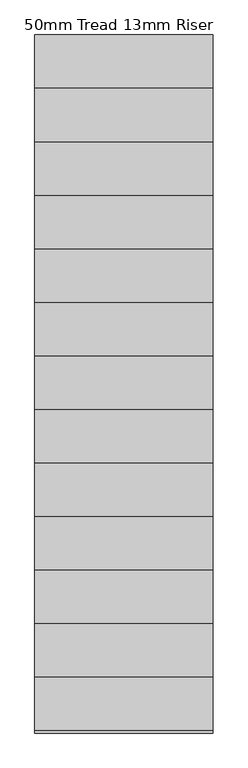
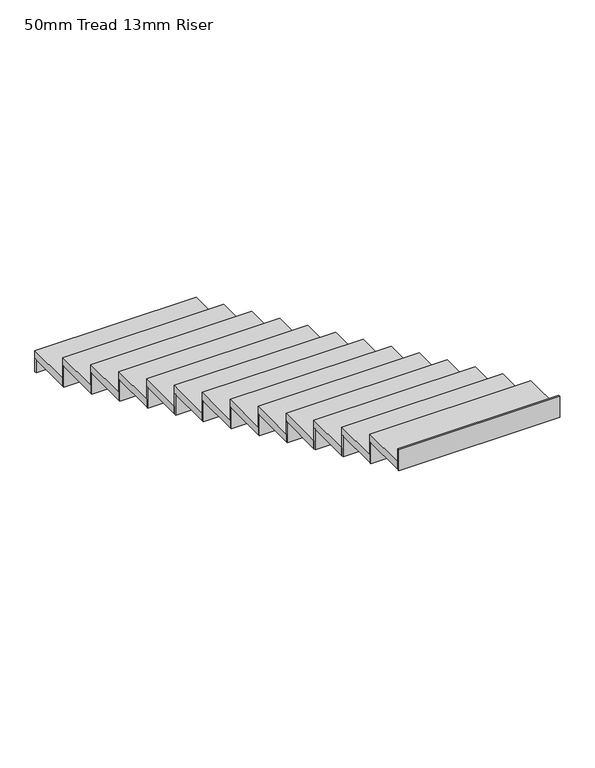
"""IFC4 building model written with IfcOpenShell, lengths in millimetres: stair flight geometry, 50mm Tread 13mm Riser."""

from ifc_helpers import new_model, si_unit, frame, origin, origin_with_axes, place, context, project, spatial, polyline, outline, extrude, source, transform, mapped, element, save


def stair_flight_50mm_tread_13mm_riser_fee8950f(model_context):
    return source(origin(), model_context, "Body", "SweptSolid", [
        extrude(outline(polyline([(-14281.6736899, 1715.8603727), (-14281.6736899, 1728.3603727), (-13281.6736899, 1728.3603727), (-13281.6736899, 1715.8603727), (-14281.6736899, 1715.8603727)])), origin_with_axes(), (0.0, 0.0, 1.0), 86.3636364),
        extrude(outline(polyline([(-13281.6736899, 1428.3603727), (-14281.6736899, 1428.3603727), (-14281.6736899, 1728.3603727), (-13281.6736899, 1728.3603727), (-13281.6736899, 1428.3603727)])), frame((0.0, 0.0, 86.3636364), z_axis=(0.0, 0.0, 1.0), x_axis=(1.0, 0.0, 0.0)), (0.0, 0.0, 1.0), 50.0),
        extrude(outline(polyline([(-14281.6736899, 1415.8603727), (-14281.6736899, 1428.3603727), (-13281.6736899, 1428.3603727), (-13281.6736899, 1415.8603727), (-14281.6736899, 1415.8603727)])), frame((0.0, 0.0, 86.3636364), z_axis=(0.0, 0.0, 1.0), x_axis=(1.0, 0.0, 0.0)), (0.0, 0.0, 1.0), 136.3636364),
        extrude(outline(polyline([(-13281.6736899, 1128.3603727), (-14281.6736899, 1128.3603727), (-14281.6736899, 1428.3603727), (-13281.6736899, 1428.3603727), (-13281.6736899, 1128.3603727)])), frame((0.0, 0.0, 222.7272727), z_axis=(0.0, 0.0, 1.0), x_axis=(1.0, 0.0, 0.0)), (0.0, 0.0, 1.0), 50.0),
        extrude(outline(polyline([(-14281.6736899, 1115.8603727), (-14281.6736899, 1128.3603727), (-13281.6736899, 1128.3603727), (-13281.6736899, 1115.8603727), (-14281.6736899, 1115.8603727)])), frame((0.0, 0.0, 222.7272727), z_axis=(0.0, 0.0, 1.0), x_axis=(1.0, 0.0, 0.0)), (0.0, 0.0, 1.0), 136.3636364),
        extrude(outline(polyline([(-13281.6736899, 828.3603727), (-14281.6736899, 828.3603727), (-14281.6736899, 1128.3603727), (-13281.6736899, 1128.3603727), (-13281.6736899, 828.3603727)])), frame((0.0, 0.0, 359.0909091), z_axis=(0.0, 0.0, 1.0), x_axis=(1.0, 0.0, 0.0)), (0.0, 0.0, 1.0), 50.0),
        extrude(outline(polyline([(-14281.6736899, 815.8603727), (-14281.6736899, 828.3603727), (-13281.6736899, 828.3603727), (-13281.6736899, 815.8603727), (-14281.6736899, 815.8603727)])), frame((0.0, 0.0, 359.0909091), z_axis=(0.0, 0.0, 1.0), x_axis=(1.0, 0.0, 0.0)), (0.0, 0.0, 1.0), 136.3636364),
        extrude(outline(polyline([(-13281.6736899, 528.3603727), (-14281.6736899, 528.3603727), (-14281.6736899, 828.3603727), (-13281.6736899, 828.3603727), (-13281.6736899, 528.3603727)])), frame((0.0, 0.0, 495.4545455), z_axis=(0.0, 0.0, 1.0), x_axis=(1.0, 0.0, 0.0)), (0.0, 0.0, 1.0), 50.0),
        extrude(outline(polyline([(-14281.6736899, 515.8603727), (-14281.6736899, 528.3603727), (-13281.6736899, 528.3603727), (-13281.6736899, 515.8603727), (-14281.6736899, 515.8603727)])), frame((0.0, 0.0, 495.4545455), z_axis=(0.0, 0.0, 1.0), x_axis=(1.0, 0.0, 0.0)), (0.0, 0.0, 1.0), 136.3636364),
        extrude(outline(polyline([(-13281.6736899, 228.3603727), (-14281.6736899, 228.3603727), (-14281.6736899, 528.3603727), (-13281.6736899, 528.3603727), (-13281.6736899, 228.3603727)])), frame((0.0, 0.0, 631.8181818), z_axis=(0.0, 0.0, 1.0), x_axis=(1.0, 0.0, 0.0)), (0.0, 0.0, 1.0), 50.0),
        extrude(outline(polyline([(-14281.6736899, 215.8603727), (-14281.6736899, 228.3603727), (-13281.6736899, 228.3603727), (-13281.6736899, 215.8603727), (-14281.6736899, 215.8603727)])), frame((0.0, 0.0, 631.8181818), z_axis=(0.0, 0.0, 1.0), x_axis=(1.0, 0.0, 0.0)), (0.0, 0.0, 1.0), 136.3636364),
        extrude(outline(polyline([(-13281.6736899, -71.6396273), (-14281.6736899, -71.6396273), (-14281.6736899, 228.3603727), (-13281.6736899, 228.3603727), (-13281.6736899, -71.6396273)])), frame((0.0, 0.0, 768.1818182), z_axis=(0.0, 0.0, 1.0), x_axis=(1.0, 0.0, 0.0)), (0.0, 0.0, 1.0), 50.0),
        extrude(outline(polyline([(-14281.6736899, -84.1396273), (-14281.6736899, -71.6396273), (-13281.6736899, -71.6396273), (-13281.6736899, -84.1396273), (-14281.6736899, -84.1396273)])), frame((0.0, 0.0, 768.1818182), z_axis=(0.0, 0.0, 1.0), x_axis=(1.0, 0.0, 0.0)), (0.0, 0.0, 1.0), 136.3636364),
        extrude(outline(polyline([(-13281.6736899, -371.6396273), (-14281.6736899, -371.6396273), (-14281.6736899, -71.6396273), (-13281.6736899, -71.6396273), (-13281.6736899, -371.6396273)])), frame((0.0, 0.0, 904.5454545), z_axis=(0.0, 0.0, 1.0), x_axis=(1.0, 0.0, 0.0)), (0.0, 0.0, 1.0), 50.0),
        extrude(outline(polyline([(-14281.6736899, -384.1396273), (-14281.6736899, -371.6396273), (-13281.6736899, -371.6396273), (-13281.6736899, -384.1396273), (-14281.6736899, -384.1396273)])), frame((0.0, 0.0, 904.5454545), z_axis=(0.0, 0.0, 1.0), x_axis=(1.0, 0.0, 0.0)), (0.0, 0.0, 1.0), 136.3636364),
        extrude(outline(polyline([(-13281.6736899, -671.6396273), (-14281.6736899, -671.6396273), (-14281.6736899, -371.6396273), (-13281.6736899, -371.6396273), (-13281.6736899, -671.6396273)])), frame((0.0, 0.0, 1040.9090909), z_axis=(0.0, 0.0, 1.0), x_axis=(1.0, 0.0, 0.0)), (0.0, 0.0, 1.0), 50.0),
        extrude(outline(polyline([(-14281.6736899, -684.1396273), (-14281.6736899, -671.6396273), (-13281.6736899, -671.6396273), (-13281.6736899, -684.1396273), (-14281.6736899, -684.1396273)])), frame((0.0, 0.0, 1040.9090909), z_axis=(0.0, 0.0, 1.0), x_axis=(1.0, 0.0, 0.0)), (0.0, 0.0, 1.0), 136.3636364),
        extrude(outline(polyline([(-13281.6736899, -971.6396273), (-14281.6736899, -971.6396273), (-14281.6736899, -671.6396273), (-13281.6736899, -671.6396273), (-13281.6736899, -971.6396273)])), frame((0.0, 0.0, 1177.2727273), z_axis=(0.0, 0.0, 1.0), x_axis=(1.0, 0.0, 0.0)), (0.0, 0.0, 1.0), 50.0),
        extrude(outline(polyline([(-14281.6736899, -984.1396273), (-14281.6736899, -971.6396273), (-13281.6736899, -971.6396273), (-13281.6736899, -984.1396273), (-14281.6736899, -984.1396273)])), frame((0.0, 0.0, 1177.2727273), z_axis=(0.0, 0.0, 1.0), x_axis=(1.0, 0.0, 0.0)), (0.0, 0.0, 1.0), 136.3636364),
        extrude(outline(polyline([(-13281.6736899, -1271.6396273), (-14281.6736899, -1271.6396273), (-14281.6736899, -971.6396273), (-13281.6736899, -971.6396273), (-13281.6736899, -1271.6396273)])), frame((0.0, 0.0, 1313.6363636), z_axis=(0.0, 0.0, 1.0), x_axis=(1.0, 0.0, 0.0)), (0.0, 0.0, 1.0), 50.0),
        extrude(outline(polyline([(-14281.6736899, -1284.1396273), (-14281.6736899, -1271.6396273), (-13281.6736899, -1271.6396273), (-13281.6736899, -1284.1396273), (-14281.6736899, -1284.1396273)])), frame((0.0, 0.0, 1313.6363636), z_axis=(0.0, 0.0, 1.0), x_axis=(1.0, 0.0, 0.0)), (0.0, 0.0, 1.0), 136.3636364),
        extrude(outline(polyline([(-13281.6736899, -1571.6396273), (-14281.6736899, -1571.6396273), (-14281.6736899, -1271.6396273), (-13281.6736899, -1271.6396273), (-13281.6736899, -1571.6396273)])), frame((0.0, 0.0, 1450.0), z_axis=(0.0, 0.0, 1.0), x_axis=(1.0, 0.0, 0.0)), (0.0, 0.0, 1.0), 50.0),
        extrude(outline(polyline([(-14281.6736899, -1584.1396273), (-14281.6736899, -1571.6396273), (-13281.6736899, -1571.6396273), (-13281.6736899, -1584.1396273), (-14281.6736899, -1584.1396273)])), frame((0.0, 0.0, 1450.0), z_axis=(0.0, 0.0, 1.0), x_axis=(1.0, 0.0, 0.0)), (0.0, 0.0, 1.0), 136.3636364),
        extrude(outline(polyline([(-13281.6736899, -1871.6396273), (-14281.6736899, -1871.6396273), (-14281.6736899, -1571.6396273), (-13281.6736899, -1571.6396273), (-13281.6736899, -1871.6396273)])), frame((0.0, 0.0, 1586.3636364), z_axis=(0.0, 0.0, 1.0), x_axis=(1.0, 0.0, 0.0)), (0.0, 0.0, 1.0), 50.0),
        extrude(outline(polyline([(-14281.6736899, -1884.1396273), (-14281.6736899, -1871.6396273), (-13281.6736899, -1871.6396273), (-13281.6736899, -1884.1396273), (-14281.6736899, -1884.1396273)])), frame((0.0, 0.0, 1586.3636364), z_axis=(0.0, 0.0, 1.0), x_axis=(1.0, 0.0, 0.0)), (0.0, 0.0, 1.0), 136.3636364),
        extrude(outline(polyline([(-14281.6736899, -2184.1396273), (-14281.6736899, -2171.6396273), (-13281.6736899, -2171.6396273), (-13281.6736899, -2184.1396273), (-14281.6736899, -2184.1396273)])), frame((0.0, 0.0, 1722.7272727), z_axis=(0.0, 0.0, 1.0), x_axis=(1.0, 0.0, 0.0)), (0.0, 0.0, 1.0), 136.3636364),
        extrude(outline(polyline([(-13281.6736899, -2171.6396273), (-14281.6736899, -2171.6396273), (-14281.6736899, -1871.6396273), (-13281.6736899, -1871.6396273), (-13281.6736899, -2171.6396273)])), frame((0.0, 0.0, 1722.7272727), z_axis=(0.0, 0.0, 1.0), x_axis=(1.0, 0.0, 0.0)), (0.0, 0.0, 1.0), 50.0),
    ])


if __name__ == "__main__":
    model = new_model("IFC4")
    model_context = context("Model", 3, world=origin())
    ifc_project = project(units=[si_unit("LENGTHUNIT", "METRE", prefix="MILLI")], contexts=[model_context])
    site = spatial("IfcSite", under=ifc_project)
    building = spatial("IfcBuilding", under=site)
    placement = place(None, origin())
    stair_flight_50mm_tread_13mm_riser_shape = stair_flight_50mm_tread_13mm_riser_fee8950f(model_context)
    element("IfcStairFlight", 1, ObjectType="50mm Tread 13mm Riser", at=placement, inside=building, context=model_context, shape_type="MappedRepresentation", body=[
        mapped(stair_flight_50mm_tread_13mm_riser_shape, transform((0.0, 0.0, 0.0), x_axis=(1.0, 0.0, 0.0), y_axis=(0.0, 1.0, 0.0), z_axis=(0.0, 0.0, 1.0))),
    ])
    save(model, "model.ifc")
